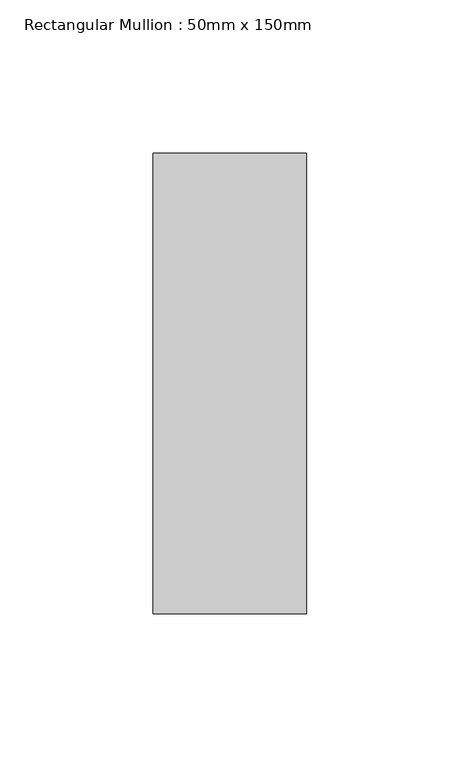
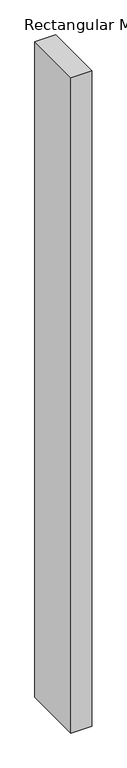
"""IFC4 building model written with IfcOpenShell, lengths in millimetres: member geometry, Rectangular Mullion : 50mm x 150mm."""

from ifc_helpers import new_model, si_unit, frame, origin, place, context, project, spatial, polyline, outline, extrude, source, transform, mapped, element, save


def rectangular_mullion_50mm_x_150mm_06590005(model_context):
    return source(origin(), model_context, "Body", "SweptSolid", [
        extrude(outline(polyline([(25.0, 75.0), (25.0, -75.0), (-25.0, -75.0), (-25.0, 75.0), (25.0, 75.0)])), frame((0.0, 0.0, -1665.0), z_axis=(0.0, 0.0, 1.0), x_axis=(1.0, 0.0, 0.0)), (0.0, 0.0, 1.0), 1665.0),
    ])


if __name__ == "__main__":
    model = new_model("IFC4")
    model_context = context("Model", 3, world=origin())
    ifc_project = project(units=[si_unit("LENGTHUNIT", "METRE", prefix="MILLI")], contexts=[model_context])
    site = spatial("IfcSite", under=ifc_project)
    building = spatial("IfcBuilding", under=site)
    placement = place(None, origin())
    rectangular_mullion_50mm_x_150mm_shape = rectangular_mullion_50mm_x_150mm_06590005(model_context)
    element("IfcMember", 1, ObjectType="Rectangular Mullion : 50mm x 150mm", at=placement, inside=building, context=model_context, shape_type="MappedRepresentation", body=[
        mapped(rectangular_mullion_50mm_x_150mm_shape, transform((0.0, 0.0, 0.0), x_axis=(1.0, 0.0, 0.0), y_axis=(0.0, 1.0, 0.0), z_axis=(0.0, 0.0, 1.0))),
    ])
    save(model, "model.ifc")

# Revit data of these elements
# Type "Rectangular Mullion : 50mm x 150mm"
#   built-in parameter 1007304 = 0.492126 (stored number, unit not read)
#   built-in parameter 1007301 = 0.082021 (stored number, unit not read)
#   built-in parameter 1007300 = 0.082021 (stored number, unit not read)
# Element 1 (IfcMember, "Rectangular Mullion : 50mm x 150mm")
#   Materials on its faces: "Aluminum"
# Materials
#   "Aluminum": class "Metal", colour RGB 244 244 244, transparency 0, Description = "Aluminum 6061", Cost = 0
